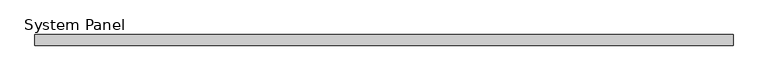
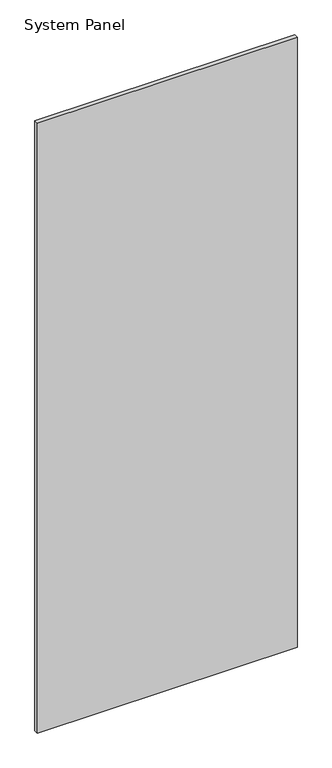
"""IFC4 building model written with IfcOpenShell, lengths in millimetres: plate geometry, System Panel : WWm-Glass-20mm-10mmOffset."""

from ifc_helpers import new_model, si_unit, origin, origin_with_axes, place, context, project, spatial, polyline, outline, extrude, source, transform, mapped, element, save


def system_panel_ceb25e36(model_context):
    return source(origin(), model_context, "Body", "SweptSolid", [
        extrude(outline(polyline([(634.5, 0.0), (-634.5, 0.0), (-634.5, 20.0), (634.5, 20.0), (634.5, 0.0)])), origin_with_axes(), (0.0, 0.0, 1.0), 3150.0),
    ])


if __name__ == "__main__":
    model = new_model("IFC4")
    model_context = context("Model", 3, world=origin())
    ifc_project = project(units=[si_unit("LENGTHUNIT", "METRE", prefix="MILLI")], contexts=[model_context])
    site = spatial("IfcSite", under=ifc_project)
    building = spatial("IfcBuilding", under=site)
    placement = place(None, origin())
    system_panel_shape = system_panel_ceb25e36(model_context)
    element("IfcPlate", 1, ObjectType="System Panel : WWm-Glass-20mm-10mmOffset", at=placement, inside=building, context=model_context, shape_type="MappedRepresentation", body=[
        mapped(system_panel_shape, transform((0.0, 0.0, 0.0), x_axis=(1.0, 0.0, 0.0), y_axis=(0.0, 1.0, 0.0), z_axis=(0.0, 0.0, 1.0))),
    ])
    save(model, "model.ifc")

# Revit data of these elements
# Type "System Panel : WWm-Glass-20mm-10mmOffset"
#   Finish = ""
# Element 1 (IfcPlate, "System Panel : WWm-Glass-20mm-10mmOffset")
#   Materials on its faces: "WW-EC-GL-Storefront"
# Materials
#   "WW-EC-GL-Storefront": class "Glass", colour RGB 236 240 239, transparency 0.85, Description = "Storefront Glass", Cost = 0
